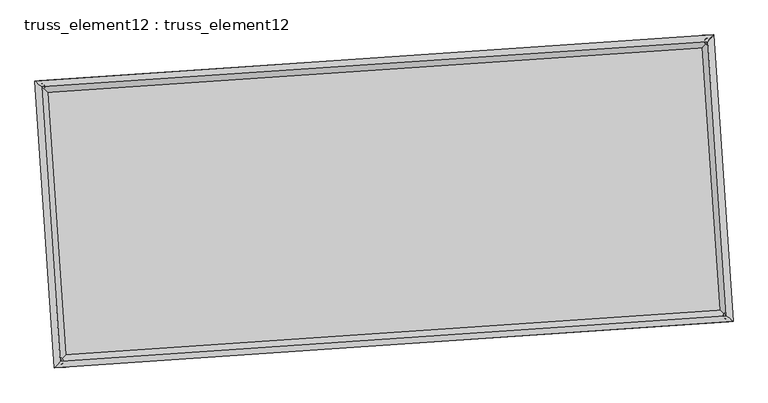
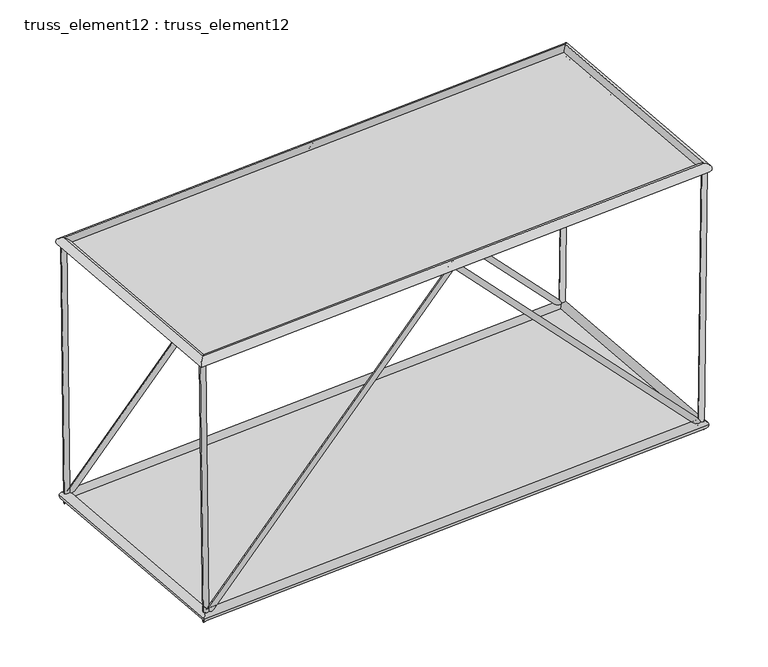
"""IFC4 building model written with IfcOpenShell, lengths in millimetres: plate geometry, truss_element12 : truss_element12."""

from ifc_helpers import new_model, si_unit, frame, origin, origin_with_axes, place, context, project, spatial, polyline, circle_curve, ellipse_curve, outline, extrude, source, transform, mapped, element, save
from ifc_brep_helpers import plane_surface, cylinder_surface, advanced_brep


def truss_element12_truss_element12_8f72c4cc(model_context):
    return source(origin(), model_context, "Body", "SolidModel", [
        advanced_brep(
        [(-3727.2192532, 2271.9774942, 5000.2332074), (-3826.3148624, 2258.6167835, 4998.9875555), (-3666.4649033, 2276.1201024, 122.5964802), (-3762.5219795, 2262.9665777, -122.5964802), (1064.2915004, 2598.6923983, 5071.7241835), (1064.7311595, 2592.1186192, 4927.4822392), (5793.9313565, 2921.188561, 122.5885273), (5890.8296205, 2921.1919275, -122.5885273), (5855.7938545, 2925.4067296, 5000.230225), (5955.7855808, 2925.6210275, 4998.9618575)],
        [
            (0, 1, circle_curve(frame((-3776.7670578, 2265.2971389, 4999.6103815), z_axis=(-0.012454723282468943, -0.0008492402357976954, 0.9999220762934375), x_axis=(-0.1336072742715059, 0.9910340154549612, -0.0008224797592794459)), 50.0)),
            (1, 0, circle_curve(frame((-3776.7670578, 2265.2971389, 4999.6103815), z_axis=(-0.012454723282468943, -0.0008492402357976954, 0.9999220762934375), x_axis=(-0.1336072742715059, 0.9910340154549612, -0.0008224797592794459)), 50.0)),
            (0, 2),
            (2, 3, ellipse_curve(frame((-3714.4934414, 2269.54334, 0.0), z_axis=(-0.9280745157714434, -0.06328187328893568, 0.36697833408614733), x_axis=(0.3661281906369683, 0.02496488953598211, 0.9302294890570586)), 132.0786249, 50.0)),
            (3, 1),
            (3, 2, ellipse_curve(frame((-3714.4934414, 2269.54334, 0.0), z_axis=(-0.9280745157714434, -0.06328187328893568, 0.36697833408614733), x_axis=(0.3661281906369683, 0.02496488953598211, 0.9302294890570586)), 132.0786249, 50.0)),
            (2, 4),
            (4, 5, ellipse_curve(frame((1064.5113299, 2595.4055087, 4999.6032114), z_axis=(-0.9976833943172301, -0.06802823810885233, 5.935870352728737e-05), x_axis=(-5.9221192921833396e-05, -4.03806802274625e-06, -0.9999999982382721)), 72.2780144, 50.0)),
            (5, 3),
            (5, 4, ellipse_curve(frame((1064.5113299, 2595.4055087, 4999.6032114), z_axis=(-0.9976833943172301, -0.06802823810885233, 5.935870352728737e-05), x_axis=(-5.9221192921833396e-05, -4.03806802274625e-06, -0.9999999982382721)), 72.2780144, 50.0)),
            (4, 6),
            (6, 7, ellipse_curve(frame((5842.3804885, 2921.1902443, 0.0), z_axis=(-0.9281379125811653, -0.06328619607639555, -0.36681721962805564), x_axis=(-0.3659674494172622, -0.024953929203248196, 0.9302930330730972)), 132.0610358, 50.0)),
            (7, 5),
            (7, 6, ellipse_curve(frame((5842.3804885, 2921.1902443, 0.0), z_axis=(-0.9281379125811653, -0.06328619607639555, -0.36681721962805564), x_axis=(-0.3659674494172622, -0.024953929203248196, 0.9302930330730972)), 132.0610358, 50.0)),
            (8, 9, circle_curve(frame((5905.7897177, 2925.5138785, 4999.5960413), z_axis=(0.012681845830496502, 0.0008647268589705681, 0.9999192082532424), x_axis=(-0.0021537739507081696, 0.9999973299402997, -0.0008374783822429829)), 50.0)),
            (9, 8, circle_curve(frame((5905.7897177, 2925.5138785, 4999.5960413), z_axis=(0.012681845830496502, 0.0008647268589705681, 0.9999192082532424), x_axis=(-0.0021537739507081696, 0.9999973299402997, -0.0008374783822429829)), 50.0)),
            (6, 8),
            (9, 7),
        ],
        [
            plane_surface(frame((-3776.7670578, 2315.2971208, 4999.6528468), z_axis=(-0.012454723282470215, -0.0008492402357928436, 0.9999220762934375), x_axis=(0.9999224369259634, -1.0577872589401237e-05, 0.012454718790543492))),
            cylinder_surface(frame((-3776.7670578, 2265.2971389, 4999.6103815), z_axis=(-0.012454723282468943, -0.0008492402357976954, 0.9999220762934375), x_axis=(-0.1336072742715059, 0.9910340154549612, -0.0008224797592794459)), 50.0),
            cylinder_surface(frame((-3714.4934414, 2269.54334, 0.0), z_axis=(-0.6902134913462219, -0.04706303422778228, -0.7220736854178621), x_axis=(-0.020417106549851006, 0.998752022715791, -0.04558002721859809)), 50.0),
            cylinder_surface(frame((1064.5113299, 2595.4055087, 4999.6032114), z_axis=(-0.6901279623524434, -0.04705720233082522, 0.7221558109494518), x_axis=(-0.11534915142313243, 0.9922789674463691, -0.045574379091006735)), 50.0),
            plane_surface(frame((5905.7897177, 2875.5138972, 4999.6392811), z_axis=(0.01268184583049596, 0.0008647268589738932, 0.9999192082532424), x_axis=(0.9999195821596514, -1.0967214670642978e-05, -0.012681841088291169))),
            cylinder_surface(frame((5842.3804885, 2921.1902443, 0.0), z_axis=(-0.012681845830496502, -0.0008647268589705681, -0.9999192082532424), x_axis=(-0.0021537739507081696, 0.9999973299402997, -0.0008374783822429829)), 50.0),
        ],
        [
            (0, [[1, 2]]),
            (1, [[-1, 3, 4, 5]]),
            (1, [[-2, -5, 6, -3]]),
            (2, [[-4, 7, 8, 9]]),
            (2, [[-6, -9, 10, -7]]),
            (3, [[-8, 11, 12, 13]]),
            (3, [[-10, -13, 14, -11]]),
            (4, [[15, 16]]),
            (5, [[-12, 17, -16, 18]]),
            (5, [[-14, -18, -15, -17]]),
        ],
    ),
        advanced_brep(
        [(-3455.1063003, -1718.7560901, 5000.2332074), (-3554.2019095, -1732.1168008, 4998.9875555), (-3394.3519504, -1714.6134819, 122.5964802), (-3490.4090266, -1727.7670066, -122.5964802), (1336.4044533, -1392.041186, 5071.7241835), (1336.8441124, -1398.6149651, 4927.4822392), (6066.0443094, -1069.5450233, 122.5885273), (6162.9425734, -1069.5416568, -122.5885273), (6127.9068074, -1065.3268547, 5000.230225), (6227.8985337, -1065.1125568, 4998.9618575)],
        [
            (0, 1, circle_curve(frame((-3504.6541049, -1725.4364454, 4999.6103815), z_axis=(-0.012454723282468884, -0.0008492402357977014, 0.9999220762934377), x_axis=(-0.13360727427150593, 0.9910340154549612, -0.0008224797592794322)), 50.0)),
            (1, 0, circle_curve(frame((-3504.6541049, -1725.4364454, 4999.6103815), z_axis=(-0.012454723282468884, -0.0008492402357977014, 0.9999220762934377), x_axis=(-0.13360727427150593, 0.9910340154549612, -0.0008224797592794322)), 50.0)),
            (0, 2),
            (2, 3, ellipse_curve(frame((-3442.3804885, -1721.1902443, 0.0), z_axis=(-0.9280745157714434, -0.06328187328893571, 0.3669783340861473), x_axis=(0.36612819063696816, 0.024964889535982103, 0.9302294890570585)), 132.0786249, 50.0)),
            (3, 1),
            (3, 2, ellipse_curve(frame((-3442.3804885, -1721.1902443, 0.0), z_axis=(-0.9280745157714434, -0.06328187328893571, 0.3669783340861473), x_axis=(0.36612819063696816, 0.024964889535982103, 0.9302294890570585)), 132.0786249, 50.0)),
            (2, 4),
            (4, 5, ellipse_curve(frame((1336.6242828, -1395.3280756, 4999.6032114), z_axis=(-0.9976833943172301, -0.0680282381088523, 5.9358703526404644e-05), x_axis=(-5.9221192920910944e-05, -4.0380680227270335e-06, -0.9999999982382721)), 72.2780144, 50.0)),
            (5, 3),
            (5, 4, ellipse_curve(frame((1336.6242828, -1395.3280756, 4999.6032114), z_axis=(-0.9976833943172301, -0.0680282381088523, 5.9358703526404644e-05), x_axis=(-5.9221192920910944e-05, -4.0380680227270335e-06, -0.9999999982382721)), 72.2780144, 50.0)),
            (4, 6),
            (6, 7, ellipse_curve(frame((6114.4934414, -1069.54334, 0.0), z_axis=(-0.9281379125811651, -0.06328619607639552, -0.36681721962805613), x_axis=(-0.3659674494172627, -0.024953929203248182, 0.9302930330730971)), 132.0610358, 50.0)),
            (7, 5),
            (7, 6, ellipse_curve(frame((6114.4934414, -1069.54334, 0.0), z_axis=(-0.9281379125811651, -0.06328619607639552, -0.36681721962805613), x_axis=(-0.3659674494172627, -0.024953929203248182, 0.9302930330730971)), 132.0610358, 50.0)),
            (8, 9, circle_curve(frame((6177.9026706, -1065.2197058, 4999.5960413), z_axis=(0.01268184583049621, 0.0008647268589706002, 0.9999192082532423), x_axis=(-0.002153773950708037, 0.9999973299402997, -0.0008374783822430173)), 50.0)),
            (9, 8, circle_curve(frame((6177.9026706, -1065.2197058, 4999.5960413), z_axis=(0.01268184583049621, 0.0008647268589706002, 0.9999192082532423), x_axis=(-0.002153773950708037, 0.9999973299402997, -0.0008374783822430173)), 50.0)),
            (6, 8),
            (9, 7),
        ],
        [
            plane_surface(frame((-3504.6541049, -1675.4364635, 4999.6528468), z_axis=(-0.012454723282470215, -0.0008492402357928367, 0.9999220762934375), x_axis=(0.9999224369259634, -1.0577872589401237e-05, 0.012454718790543492))),
            cylinder_surface(frame((-3504.6541049, -1725.4364454, 4999.6103815), z_axis=(-0.012454723282468884, -0.0008492402357977014, 0.9999220762934377), x_axis=(-0.13360727427150593, 0.9910340154549612, -0.0008224797592794322)), 50.0),
            cylinder_surface(frame((-3442.3804885, -1721.1902443, 0.0), z_axis=(-0.6902134913462216, -0.04706303422778227, -0.7220736854178624), x_axis=(-0.020417106549850947, 0.998752022715791, -0.04558002721859812)), 50.0),
            cylinder_surface(frame((1336.6242828, -1395.3280756, 4999.6032114), z_axis=(-0.6901279623524446, -0.04705720233082525, 0.722155810949451), x_axis=(-0.11534915142313235, 0.9922789674463693, -0.04557437909100684)), 50.0),
            plane_surface(frame((6177.9026706, -1115.2196871, 4999.6392811), z_axis=(0.01268184583049596, 0.0008647268589738886, 0.9999192082532424), x_axis=(0.9999195821596514, -1.0967214670642978e-05, -0.012681841088291169))),
            cylinder_surface(frame((6114.4934414, -1069.54334, 0.0), z_axis=(-0.01268184583049621, -0.0008647268589706002, -0.9999192082532423), x_axis=(-0.002153773950708037, 0.9999973299402997, -0.0008374783822430173)), 50.0),
        ],
        [
            (0, [[1, 2]]),
            (1, [[-1, 3, 4, 5]]),
            (1, [[-2, -5, 6, -3]]),
            (2, [[-4, 7, 8, 9]]),
            (2, [[-6, -9, 10, -7]]),
            (3, [[-8, 11, 12, 13]]),
            (3, [[-10, -13, 14, -11]]),
            (4, [[15, 16]]),
            (5, [[-12, 17, -16, 18]]),
            (5, [[-14, -18, -15, -17]]),
        ],
    ),
        advanced_brep(
        [(-3504.657868, -1725.4406162, 4909.6103816), (-3504.6503418, -1725.4322746, 5089.6103814), (-3776.7627634, 2265.2935175, 5089.6103814), (-3776.7713523, 2265.3007603, 4909.6103816), (5905.7862199, 2925.5097258, 5089.5960412), (5905.7932154, 2925.5180313, 4909.5960413), (6177.8986415, -1065.2160663, 5089.5960412), (6177.9066997, -1065.2233452, 4909.5960413)],
        [
            (0, 1, ellipse_curve(frame((-3504.6541049, -1725.4364454, 4999.6103815), z_axis=(-0.7535719234046849, 0.6573654662781367, 1.0448235056074835e-06), x_axis=(-0.6573654662773142, -0.7535719234054024, 1.0448234933563717e-06)), 127.2792206, 90.0)),
            (1, 2),
            (2, 3, ellipse_curve(frame((-3776.7670578, 2265.2971389, 4999.6103815), z_axis=(-0.6573654662773138, -0.7535719234054027, 1.0448234939876744e-06), x_axis=(0.753571923404685, -0.6573654662781364, -1.044823506238787e-06)), 127.2792206, 90.0)),
            (3, 0),
            (1, 0, ellipse_curve(frame((-3504.6541049, -1725.4364454, 4999.6103815), z_axis=(-0.7535719234046849, 0.6573654662781367, 1.0448235056074835e-06), x_axis=(-0.6573654662773142, -0.7535719234054024, 1.0448234933563717e-06)), 127.2792206, 90.0)),
            (3, 2, ellipse_curve(frame((-3776.7670578, 2265.2971389, 4999.6103815), z_axis=(-0.6573654662773138, -0.7535719234054027, 1.0448234939876744e-06), x_axis=(0.753571923404685, -0.6573654662781364, -1.044823506238787e-06)), 127.2792206, 90.0)),
            (2, 4),
            (4, 5, ellipse_curve(frame((5905.7897177, 2925.5138785, 4999.5960413), z_axis=(-0.7535719234046856, 0.657365466278136, 1.0448235047075032e-06), x_axis=(-0.6573654662773132, -0.7535719234054032, 1.0448234955189582e-06)), 127.2792206, 90.0)),
            (5, 3),
            (5, 4, ellipse_curve(frame((5905.7897177, 2925.5138785, 4999.5960413), z_axis=(-0.7535719234046856, 0.657365466278136, 1.0448235047075032e-06), x_axis=(-0.6573654662773132, -0.7535719234054032, 1.0448234955189582e-06)), 127.2792206, 90.0)),
            (4, 6),
            (6, 7, ellipse_curve(frame((6177.9026706, -1065.2197058, 4999.5960413), z_axis=(0.6573654662773132, 0.7535719234054032, -1.0448234948876552e-06), x_axis=(-0.7535719234046856, 0.6573654662781359, 1.0448235040762e-06)), 127.2792206, 90.0)),
            (7, 5),
            (7, 6, ellipse_curve(frame((6177.9026706, -1065.2197058, 4999.5960413), z_axis=(0.6573654662773132, 0.7535719234054032, -1.0448234948876552e-06), x_axis=(-0.7535719234046856, 0.6573654662781359, 1.0448235040762e-06)), 127.2792206, 90.0)),
            (6, 1),
            (0, 7),
        ],
        [
            cylinder_surface(frame((-3504.6541049, -1725.4364454, 4999.6103815), z_axis=(0.06802823822869772, -0.9976833960748768, 0.0), x_axis=(-0.9976833950706322, -0.06802823816022209, 4.4868174597883384e-05)), 90.0),
            cylinder_surface(frame((-3776.7670578, 2265.2971389, 4999.6103815), z_axis=(-0.997683396073788, -0.06802823822862193, 1.4776035641462583e-06), x_axis=(-0.06802823810069086, 0.9976833951400486, 4.339057104379111e-05)), 90.0),
            cylinder_surface(frame((5905.7897177, 2925.5138785, 4999.5960413), z_axis=(-0.06802823822869962, 0.9976833960748769, 0.0), x_axis=(0.9976833951985631, 0.06802823816894711, 4.1912967474538696e-05)), 90.0),
            cylinder_surface(frame((6177.9026706, -1065.2197058, 4999.5960413), z_axis=(0.9976833960737879, 0.06802823822862185, -1.4776035632534604e-06), x_axis=(0.06802823822862185, -0.9976833951313253, 4.339057102990407e-05)), 90.0),
        ],
        [
            (0, [[1, 2, 3, 4]]),
            (0, [[5, -4, 6, -2]]),
            (1, [[-3, 7, 8, 9]]),
            (1, [[-6, -9, 10, -7]]),
            (2, [[-8, 11, 12, 13]]),
            (2, [[-10, -13, 14, -11]]),
            (3, [[-12, 15, -1, 16]]),
            (3, [[-14, -16, -5, -15]]),
        ],
    ),
        advanced_brep(
        [(-3358.7115243, -1625.2761972, 0.0), (-3526.0494527, -1817.1042913, 0.0), (-3810.4074885, 2353.2123043, 0.0), (-3618.5793943, 2185.8743758, 0.0), (5926.0494527, 3017.1042913, 0.0), (5758.7115243, 2825.2761972, 0.0), (6210.4074885, -1153.2123043, 0.0), (6018.5793943, -985.8743758, 0.0)],
        [
            (0, 1, ellipse_curve(frame((-3442.3804885, -1721.1902443, 0.0), z_axis=(-0.7535719234054572, 0.6573654662780816, 0.0), x_axis=(-0.6573654662780816, -0.7535719234054573, 0.0)), 127.2792206, 90.0)),
            (1, 2),
            (2, 3, ellipse_curve(frame((-3714.4934414, 2269.54334, 0.0), z_axis=(-0.6573654662780816, -0.7535719234054573, 0.0), x_axis=(0.7535719234054572, -0.6573654662780816, 0.0)), 127.2792206, 90.0)),
            (3, 0),
            (1, 0, ellipse_curve(frame((-3442.3804885, -1721.1902443, 0.0), z_axis=(-0.7535719234054572, 0.6573654662780816, 0.0), x_axis=(-0.6573654662780816, -0.7535719234054573, 0.0)), 127.2792206, 90.0)),
            (3, 2, ellipse_curve(frame((-3714.4934414, 2269.54334, 0.0), z_axis=(-0.6573654662780816, -0.7535719234054573, 0.0), x_axis=(0.7535719234054572, -0.6573654662780816, 0.0)), 127.2792206, 90.0)),
            (2, 4),
            (4, 5, ellipse_curve(frame((5842.3804885, 2921.1902443, 0.0), z_axis=(-0.753571923405458, 0.6573654662780807, 0.0), x_axis=(-0.6573654662780808, -0.7535719234054579, 0.0)), 127.2792206, 90.0)),
            (5, 3),
            (5, 4, ellipse_curve(frame((5842.3804885, 2921.1902443, 0.0), z_axis=(-0.753571923405458, 0.6573654662780807, 0.0), x_axis=(-0.6573654662780808, -0.7535719234054579, 0.0)), 127.2792206, 90.0)),
            (4, 6),
            (6, 7, ellipse_curve(frame((6114.4934414, -1069.54334, 0.0), z_axis=(0.6573654662780809, 0.7535719234054579, 0.0), x_axis=(-0.753571923405458, 0.6573654662780809, 0.0)), 127.2792206, 90.0)),
            (7, 5),
            (7, 6, ellipse_curve(frame((6114.4934414, -1069.54334, 0.0), z_axis=(0.6573654662780809, 0.7535719234054579, 0.0), x_axis=(-0.753571923405458, 0.6573654662780809, 0.0)), 127.2792206, 90.0)),
            (6, 1),
            (0, 7),
        ],
        [
            cylinder_surface(frame((-3442.3804885, -1721.1902443, 0.0), z_axis=(0.06802823822870091, -0.9976833960748767, 0.0), x_axis=(-0.9976833960748767, -0.06802823822870091, 0.0)), 90.0),
            cylinder_surface(frame((-3714.4934414, 2269.54334, 0.0), z_axis=(-0.9976833960748768, -0.06802823822869955, 0.0), x_axis=(-0.06802823822869955, 0.9976833960748768, 0.0)), 90.0),
            cylinder_surface(frame((5842.3804885, 2921.1902443, 0.0), z_axis=(-0.06802823822870294, 0.9976833960748764, 0.0), x_axis=(0.9976833960748764, 0.06802823822870294, 0.0)), 90.0),
            cylinder_surface(frame((6114.4934414, -1069.54334, 0.0), z_axis=(0.9976833960748767, 0.06802823822869943, 0.0), x_axis=(0.06802823822869943, -0.9976833960748767, 0.0)), 90.0),
        ],
        [
            (0, [[1, 2, 3, 4]]),
            (0, [[5, -4, 6, -2]]),
            (1, [[-3, 7, 8, 9]]),
            (1, [[-6, -9, 10, -7]]),
            (2, [[-8, 11, 12, 13]]),
            (2, [[-10, -13, 14, -11]]),
            (3, [[-12, 15, -1, 16]]),
            (3, [[-14, -16, -5, -15]]),
        ],
    ),
        extrude(outline(polyline([(-3442.3804885, -1721.1902443), (-3714.4934414, 2269.54334), (5842.3804885, 2921.1902443), (6114.4934414, -1069.54334), (-3442.3804885, -1721.1902443)])), origin_with_axes(), (0.0, 0.0, 1.0), 20.0),
        extrude(outline(polyline([(-2000.0, 4852.5197541), (2000.0, 4852.5197541), (1999.9999999, -4852.5197541), (-2000.0000001, -4852.5197541), (-2000.0, 4852.5197541)])), frame((1200.5678064, 600.0387166, 4999.6032114), z_axis=(1.4741805425190185e-06, 1.005187586264448e-07, 0.9999999999989084), x_axis=(-0.06802823822870088, 0.9976833960748767, 0.0)), (0.0, 0.0, 1.0), 20.0),
    ])


if __name__ == "__main__":
    model = new_model("IFC4")
    model_context = context("Model", 3, world=origin())
    ifc_project = project(units=[si_unit("LENGTHUNIT", "METRE", prefix="MILLI")], contexts=[model_context])
    site = spatial("IfcSite", under=ifc_project)
    building = spatial("IfcBuilding", under=site)
    placement = place(None, origin())
    truss_element12_truss_element12_shape = truss_element12_truss_element12_8f72c4cc(model_context)
    element("IfcPlate", 1, ObjectType="truss_element12 : truss_element12", at=placement, inside=building, context=model_context, shape_type="MappedRepresentation", body=[
        mapped(truss_element12_truss_element12_shape, transform((0.0, 0.0, 0.0), x_axis=(1.0, 0.0, 0.0), y_axis=(0.0, 1.0, 0.0), z_axis=(0.0, 0.0, 1.0))),
    ])
    save(model, "model.ifc")

# Revit data of these elements
# Type "truss_element12 : truss_element12"
#   steellbar1 = 90 mm
#   steelbar2 = 50 mm
#   offset1 = 5000 mm
#   M = Default Roof
# Element 1 (IfcPlate, "truss_element12 : truss_element12")
#   Materials on its faces: "Default Roof"
# Materials
#   "Default Roof": class "Miscellaneous", colour RGB 0 127 0, transparency 0, Comments = "Rendering appearance not upgraded Rendering appearance not upgraded ", Cost = 0
